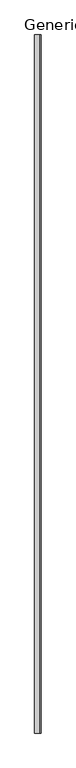
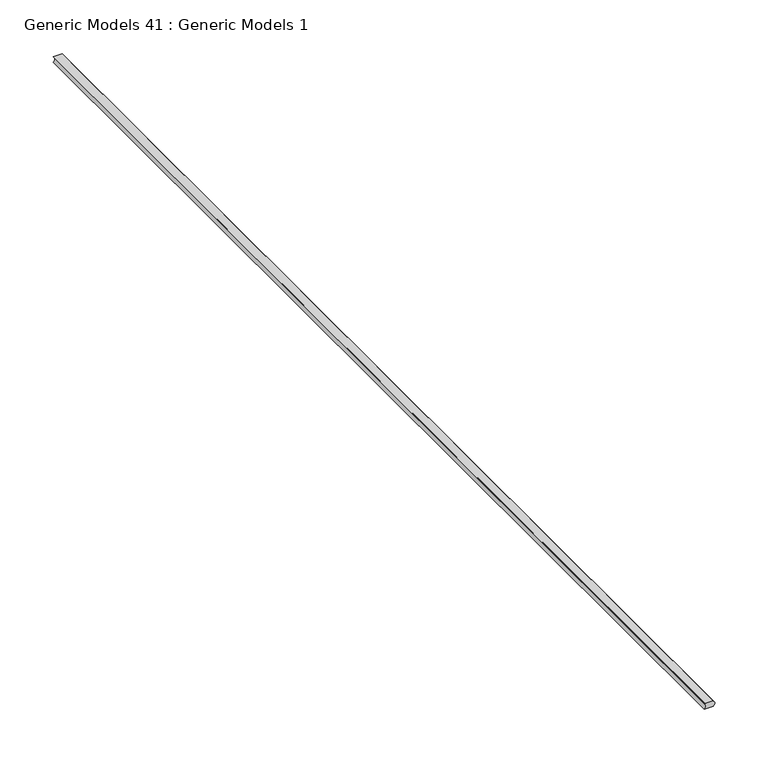
"""IFC4 building model written with IfcOpenShell, lengths in millimetres: proxy geometry, Generic Models 41 : Generic Models 1."""

import ifcopenshell
import ifcopenshell.guid

model = None  # the IFC model being written
_history = None  # IfcOwnerHistory: only IFC2X3 demands one
_inside = {}  # id of a spatial element -> (the spatial element, [elements in it])
_under = {}  # id of a project, library or spatial element -> (it, [spatial elements below it])
_declared = {}  # id of a project -> (the project, [libraries it declares])
_typed = {}  # id of a type object -> (the type object, [elements of that type])
_made_of = {}  # id of a material, layer set ... -> (it, [elements and type objects made of it])


def new_model(schema):
    """Start an empty IFC model of exactly this schema.

    Asked for "IFC4X3", IfcOpenShell would pick the latest addendum, in which some entities
    have other attributes; the version numbers below select the first issue.
    IFC2X3 requires an IfcOwnerHistory on every rooted entity: one is made here for all.
    """
    global model, _history
    if schema == "IFC4X3":
        model = ifcopenshell.file(schema_version=(4, 3, 0, 0))
    else:
        model = ifcopenshell.file(schema=schema)
    _inside.clear()
    _under.clear()
    _declared.clear()
    _typed.clear()
    _made_of.clear()
    _history = None
    if model.schema == "IFC2X3":
        org = make("IfcOrganization", Name="unknown")
        user = make(
            "IfcPersonAndOrganization",
            ThePerson=make("IfcPerson", FamilyName="unknown"),
            TheOrganization=org,
        )
        app = make(
            "IfcApplication",
            ApplicationDeveloper=org,
            Version="unknown",
            ApplicationFullName="unknown",
            ApplicationIdentifier="unknown",
        )
        _history = make(
            "IfcOwnerHistory",
            OwningUser=user,
            OwningApplication=app,
            ChangeAction="ADDED",
            CreationDate=0,
        )
    return model


def make(cls, **values):
    """One entity of the class cls with the attributes given. An attribute that is None is left unset."""
    return model.create_entity(
        cls, **{name: value for name, value in values.items() if value is not None}
    )


def rooted(cls, **values):
    """An entity with a GlobalId (a new one), such as an element, a storey or a relation."""
    return make(cls, GlobalId=ifcopenshell.guid.new(), OwnerHistory=_history, **values)


def si_unit(unit_type, name, prefix=None):
    """IfcSIUnit, for example si_unit("LENGTHUNIT", "METRE", prefix="MILLI")."""
    return make("IfcSIUnit", UnitType=unit_type, Prefix=prefix, Name=name)


def assignment(units):
    """IfcUnitAssignment: the units of a project."""
    return None if units is None else make("IfcUnitAssignment", Units=units)


def point(xyz):
    """IfcCartesianPoint."""
    return None if xyz is None else make("IfcCartesianPoint", Coordinates=xyz)


def direction(xyz):
    """IfcDirection."""
    return None if xyz is None else make("IfcDirection", DirectionRatios=xyz)


def frame(location, z_axis=None, x_axis=None):
    """IfcAxis2Placement3D, a coordinate frame: its origin and axes. An axis left out is left unset."""
    return make(
        "IfcAxis2Placement3D",
        Location=point(location),
        Axis=direction(z_axis),
        RefDirection=direction(x_axis),
    )


def frame_2d(location, x_axis=None):
    """IfcAxis2Placement2D, a coordinate frame in the plane: its origin and x axis."""
    return make(
        "IfcAxis2Placement2D", Location=point(location), RefDirection=direction(x_axis)
    )


def origin():
    """The frame at (0, 0, 0) with its axes left unset."""
    return frame((0.0, 0.0, 0.0))


def place(relative_to, where):
    """IfcLocalPlacement: puts the frame where relative to a parent placement (None: the world)."""
    return make(
        "IfcLocalPlacement", PlacementRelTo=relative_to, RelativePlacement=where
    )


def context(
    kind, dimensions, precision=None, world=None, true_north=None, identifier=None
):
    """IfcGeometricRepresentationContext, for example the 3D "Model" context."""
    return make(
        "IfcGeometricRepresentationContext",
        ContextIdentifier=identifier,
        ContextType=kind,
        CoordinateSpaceDimension=dimensions,
        Precision=precision,
        WorldCoordinateSystem=world,
        TrueNorth=true_north,
    )


def project(units=None, contexts=None):
    """IfcProject with its units and contexts."""
    return rooted(
        "IfcProject",
        Name="project",
        RepresentationContexts=contexts,
        UnitsInContext=assignment(units),
    )


def spatial(cls, under=None, at=None, **own):
    """A site, building, storey or space (cls), placed at a placement, below another one or the project."""
    s = rooted(cls, ObjectPlacement=at, **own)
    if under is not None:
        _under.setdefault(under.id(), (under, []))[1].append(s)
    return s


def polyline(points):
    """IfcPolyline through the points."""
    return make("IfcPolyline", Points=[point(p) for p in points])


def circle_curve(where, radius):
    """IfcCircle in the frame where."""
    return make("IfcCircle", Position=where, Radius=radius)


def trimmed(basis, trim1, trim2, sense, master):
    """IfcTrimmedCurve: the piece of a basis curve between two trims."""
    return make(
        "IfcTrimmedCurve",
        BasisCurve=basis,
        Trim1=trim1,
        Trim2=trim2,
        SenseAgreement=sense,
        MasterRepresentation=master,
    )


def segment(curve, same_sense, transition):
    """IfcCompositeCurveSegment."""
    return make(
        "IfcCompositeCurveSegment",
        Transition=transition,
        SameSense=same_sense,
        ParentCurve=curve,
    )


def composite_curve(segments, self_intersect=None):
    """IfcCompositeCurve: segments joined end to end."""
    return make("IfcCompositeCurve", Segments=segments, SelfIntersect=self_intersect)


def outline(outer, holes=None, kind="AREA"):
    """IfcArbitraryClosedProfileDef: a profile drawn as a closed curve; with holes, ...WithVoids."""
    if holes is None:
        return make("IfcArbitraryClosedProfileDef", ProfileType=kind, OuterCurve=outer)
    return make(
        "IfcArbitraryProfileDefWithVoids",
        ProfileType=kind,
        OuterCurve=outer,
        InnerCurves=holes,
    )


def extrude(swept, where, along, depth):
    """IfcExtrudedAreaSolid: the profile swept, set in the frame where, extruded along a direction by depth."""
    return make(
        "IfcExtrudedAreaSolid",
        SweptArea=swept,
        Position=where,
        ExtrudedDirection=direction(along),
        Depth=depth,
    )


def shape(context_of_items, identifier, shape_type, items):
    """IfcShapeRepresentation: the items that make up one representation, for example the "Body"."""
    return make(
        "IfcShapeRepresentation",
        ContextOfItems=context_of_items,
        RepresentationIdentifier=identifier,
        RepresentationType=shape_type,
        Items=items,
    )


def source(mapping_origin, context_of_items, identifier, shape_type, items):
    """IfcRepresentationMap: a shape defined once, which mapped items show again and again."""
    return make(
        "IfcRepresentationMap",
        MappingOrigin=mapping_origin,
        MappedRepresentation=shape(context_of_items, identifier, shape_type, items),
    )


def transform(
    local_origin,
    x_axis=None,
    y_axis=None,
    z_axis=None,
    scale=None,
    scale2=None,
    scale3=None,
    uniform=True,
):
    """IfcCartesianTransformationOperator3D, or its non-uniform kind. x_axis, y_axis, z_axis: its Axis1, 2, 3."""
    if uniform:
        return make(
            "IfcCartesianTransformationOperator3D",
            Axis1=direction(x_axis),
            Axis2=direction(y_axis),
            LocalOrigin=point(local_origin),
            Scale=scale,
            Axis3=direction(z_axis),
        )
    return make(
        "IfcCartesianTransformationOperator3DnonUniform",
        Axis1=direction(x_axis),
        Axis2=direction(y_axis),
        LocalOrigin=point(local_origin),
        Scale=scale,
        Axis3=direction(z_axis),
        Scale2=scale2,
        Scale3=scale3,
    )


def mapped(mapping_source, mapping_target):
    """IfcMappedItem: shows the shape of a source again, moved by a transform."""
    return make(
        "IfcMappedItem", MappingSource=mapping_source, MappingTarget=mapping_target
    )


def made_of(thing, what):
    """Note that an element or type object is made of a material, layer set ...; save() writes the relation."""
    if what is not None:
        _made_of.setdefault(what.id(), (what, []))[1].append(thing)
    return thing


def element(
    cls,
    number,
    at=None,
    inside=None,
    cuts=None,
    type_object=None,
    material=None,
    context=None,
    identifier="Body",
    shape_type=None,
    held_by="IfcProductDefinitionShape",
    body=None,
    shapes=None,
    **own,
):
    """One element of the class cls, such as IfcWall. Its Tag is "e" and its number.

    at: its placement. inside: the storey or other place that contains it. cuts: it is an
    opening in that element (IfcRelVoidsElement). A single representation is given by context,
    identifier, shape_type and body (its items); several are given by shapes. held_by: the class
    of the entity that holds the representations. save() writes the other relations.
    """
    e = rooted(cls, Tag="e%d" % number, ObjectPlacement=at, **own)
    if body is not None:
        shapes = [shape(context, identifier, shape_type, body)]
    if shapes is not None:
        e.Representation = make(held_by, Representations=shapes)
    if inside is not None:
        _inside.setdefault(inside.id(), (inside, []))[1].append(e)
    if cuts is not None:
        rooted(
            "IfcRelVoidsElement", RelatingBuildingElement=cuts, RelatedOpeningElement=e
        )
    if type_object is not None:
        _typed.setdefault(type_object.id(), (type_object, []))[1].append(e)
    return made_of(e, material)


def aggregate(whole, parts):
    """IfcRelAggregates: a whole, such as a stair, and the parts it consists of."""
    return rooted("IfcRelAggregates", RelatingObject=whole, RelatedObjects=parts)


def save(model, path):
    """Write the relations noted so far, then the file.

    IfcRelAggregates (storeys below a building ...), IfcRelContainedInSpatialStructure (elements
    in a storey), IfcRelDefinesByType, IfcRelAssociatesMaterial and IfcRelDeclares: one each for
    every whole, place, type object, material and project.
    """
    for whole, parts in _under.values():
        aggregate(whole, parts)
    for where, things in _inside.values():
        rooted(
            "IfcRelContainedInSpatialStructure",
            RelatedElements=things,
            RelatingStructure=where,
        )
    for kind, things in _typed.values():
        rooted("IfcRelDefinesByType", RelatedObjects=things, RelatingType=kind)
    for what, things in _made_of.values():
        rooted("IfcRelAssociatesMaterial", RelatedObjects=things, RelatingMaterial=what)
    for by, libraries in _declared.values():
        rooted("IfcRelDeclares", RelatingContext=by, RelatedDefinitions=libraries)
    model.write(path)


def generic_models_41_generic_models_1_f9918aae(model_context):
    return source(origin(), model_context, "Body", "SweptSolid", [
        extrude(outline(composite_curve([segment(polyline([(0.0, 50777.775), (0.0, 50787.3)]), True, "CONTINUOUS"), segment(trimmed(circle_curve(frame_2d((3.175, 50784.3852595)), 4.3100275), [point((0.0, 50787.3))], [point((6.35, 50787.3))], False, "CARTESIAN"), True, "CONTINUOUS"), segment(polyline([(6.35, 50787.3), (6.35, 50777.775)]), True, "CONTINUOUS"), segment(trimmed(circle_curve(frame_2d((3.175, 50774.8602595)), 4.3100275), [point((6.35, 50777.775))], [point((0.0, 50777.775))], True, "CARTESIAN"), True, "CONTINUOUS")], self_intersect=False)), frame((0.0, 0.0, 0.0), z_axis=(0.0, 1.0, 0.0), x_axis=(0.0, 0.0, 1.0)), (0.0, 0.0, 1.0), 1219.2),
    ])


if __name__ == "__main__":
    model = new_model("IFC4")
    model_context = context("Model", 3, world=origin())
    ifc_project = project(units=[si_unit("LENGTHUNIT", "METRE", prefix="MILLI")], contexts=[model_context])
    site = spatial("IfcSite", under=ifc_project)
    building = spatial("IfcBuilding", under=site)
    placement = place(None, origin())
    generic_models_41_generic_models_1_shape = generic_models_41_generic_models_1_f9918aae(model_context)
    element("IfcBuildingElementProxy", 1, Name="Generic Models 41 : Generic Models 1", ObjectType="Generic Models 41 : Generic Models 1", at=placement, inside=building, context=model_context, shape_type="MappedRepresentation", body=[
        mapped(generic_models_41_generic_models_1_shape, transform((0.0, 0.0, 0.0), x_axis=(1.0, 0.0, 0.0), y_axis=(0.0, 1.0, 0.0), z_axis=(0.0, 0.0, 1.0))),
    ])
    save(model, "model.ifc")

# Revit data of these elements
# Element 1 (IfcBuildingElementProxy, "Generic Models 41 : Generic Models 1")
#   Materials on its faces: "ACOUSTICAL SEALANT"
# Materials
#   "ACOUSTICAL SEALANT": class "Unassigned", colour RGB 120 120 120, transparency 0, Cost = 0
